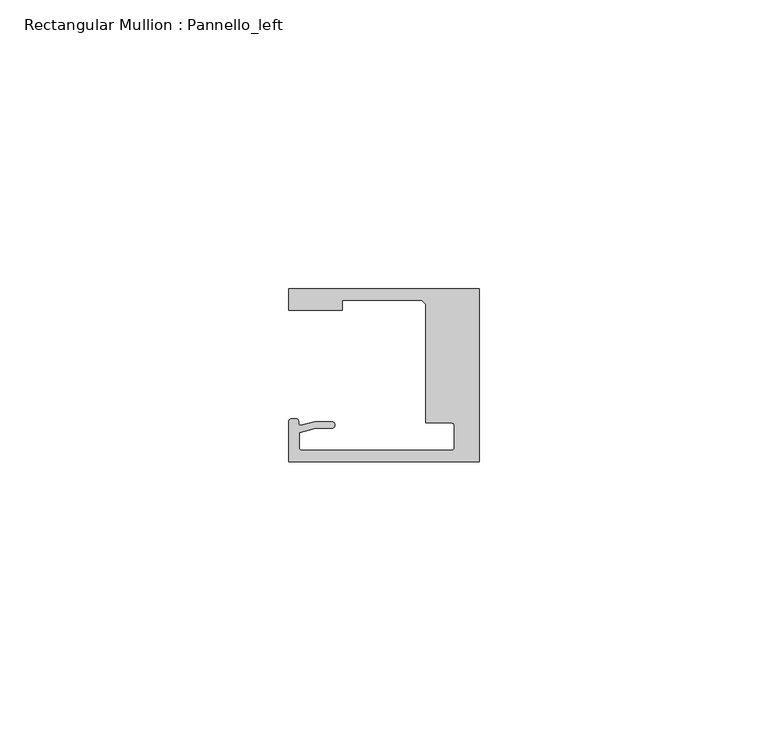
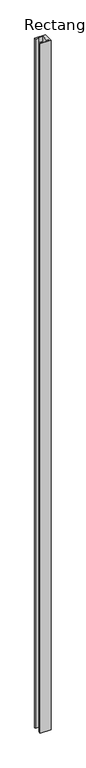
"""IFC4 building model written with IfcOpenShell, lengths in millimetres: member geometry, Rectangular Mullion : Pannello_left."""

import ifcopenshell
import ifcopenshell.guid

model = None  # the IFC model being written
_history = None  # IfcOwnerHistory: only IFC2X3 demands one
_inside = {}  # id of a spatial element -> (the spatial element, [elements in it])
_under = {}  # id of a project, library or spatial element -> (it, [spatial elements below it])
_declared = {}  # id of a project -> (the project, [libraries it declares])
_typed = {}  # id of a type object -> (the type object, [elements of that type])
_made_of = {}  # id of a material, layer set ... -> (it, [elements and type objects made of it])


def new_model(schema):
    """Start an empty IFC model of exactly this schema.

    Asked for "IFC4X3", IfcOpenShell would pick the latest addendum, in which some entities
    have other attributes; the version numbers below select the first issue.
    IFC2X3 requires an IfcOwnerHistory on every rooted entity: one is made here for all.
    """
    global model, _history
    if schema == "IFC4X3":
        model = ifcopenshell.file(schema_version=(4, 3, 0, 0))
    else:
        model = ifcopenshell.file(schema=schema)
    _inside.clear()
    _under.clear()
    _declared.clear()
    _typed.clear()
    _made_of.clear()
    _history = None
    if model.schema == "IFC2X3":
        org = make("IfcOrganization", Name="unknown")
        user = make(
            "IfcPersonAndOrganization",
            ThePerson=make("IfcPerson", FamilyName="unknown"),
            TheOrganization=org,
        )
        app = make(
            "IfcApplication",
            ApplicationDeveloper=org,
            Version="unknown",
            ApplicationFullName="unknown",
            ApplicationIdentifier="unknown",
        )
        _history = make(
            "IfcOwnerHistory",
            OwningUser=user,
            OwningApplication=app,
            ChangeAction="ADDED",
            CreationDate=0,
        )
    return model


def make(cls, **values):
    """One entity of the class cls with the attributes given. An attribute that is None is left unset."""
    return model.create_entity(
        cls, **{name: value for name, value in values.items() if value is not None}
    )


def rooted(cls, **values):
    """An entity with a GlobalId (a new one), such as an element, a storey or a relation."""
    return make(cls, GlobalId=ifcopenshell.guid.new(), OwnerHistory=_history, **values)


def si_unit(unit_type, name, prefix=None):
    """IfcSIUnit, for example si_unit("LENGTHUNIT", "METRE", prefix="MILLI")."""
    return make("IfcSIUnit", UnitType=unit_type, Prefix=prefix, Name=name)


def assignment(units):
    """IfcUnitAssignment: the units of a project."""
    return None if units is None else make("IfcUnitAssignment", Units=units)


def point(xyz):
    """IfcCartesianPoint."""
    return None if xyz is None else make("IfcCartesianPoint", Coordinates=xyz)


def direction(xyz):
    """IfcDirection."""
    return None if xyz is None else make("IfcDirection", DirectionRatios=xyz)


def frame(location, z_axis=None, x_axis=None):
    """IfcAxis2Placement3D, a coordinate frame: its origin and axes. An axis left out is left unset."""
    return make(
        "IfcAxis2Placement3D",
        Location=point(location),
        Axis=direction(z_axis),
        RefDirection=direction(x_axis),
    )


def origin():
    """The frame at (0, 0, 0) with its axes left unset."""
    return frame((0.0, 0.0, 0.0))


def place(relative_to, where):
    """IfcLocalPlacement: puts the frame where relative to a parent placement (None: the world)."""
    return make(
        "IfcLocalPlacement", PlacementRelTo=relative_to, RelativePlacement=where
    )


def context(
    kind, dimensions, precision=None, world=None, true_north=None, identifier=None
):
    """IfcGeometricRepresentationContext, for example the 3D "Model" context."""
    return make(
        "IfcGeometricRepresentationContext",
        ContextIdentifier=identifier,
        ContextType=kind,
        CoordinateSpaceDimension=dimensions,
        Precision=precision,
        WorldCoordinateSystem=world,
        TrueNorth=true_north,
    )


def project(units=None, contexts=None):
    """IfcProject with its units and contexts."""
    return rooted(
        "IfcProject",
        Name="project",
        RepresentationContexts=contexts,
        UnitsInContext=assignment(units),
    )


def spatial(cls, under=None, at=None, **own):
    """A site, building, storey or space (cls), placed at a placement, below another one or the project."""
    s = rooted(cls, ObjectPlacement=at, **own)
    if under is not None:
        _under.setdefault(under.id(), (under, []))[1].append(s)
    return s


def polyline(points):
    """IfcPolyline through the points."""
    return make("IfcPolyline", Points=[point(p) for p in points])


def circle_curve(where, radius):
    """IfcCircle in the frame where."""
    return make("IfcCircle", Position=where, Radius=radius)


def shape(context_of_items, identifier, shape_type, items):
    """IfcShapeRepresentation: the items that make up one representation, for example the "Body"."""
    return make(
        "IfcShapeRepresentation",
        ContextOfItems=context_of_items,
        RepresentationIdentifier=identifier,
        RepresentationType=shape_type,
        Items=items,
    )


def source(mapping_origin, context_of_items, identifier, shape_type, items):
    """IfcRepresentationMap: a shape defined once, which mapped items show again and again."""
    return make(
        "IfcRepresentationMap",
        MappingOrigin=mapping_origin,
        MappedRepresentation=shape(context_of_items, identifier, shape_type, items),
    )


def transform(
    local_origin,
    x_axis=None,
    y_axis=None,
    z_axis=None,
    scale=None,
    scale2=None,
    scale3=None,
    uniform=True,
):
    """IfcCartesianTransformationOperator3D, or its non-uniform kind. x_axis, y_axis, z_axis: its Axis1, 2, 3."""
    if uniform:
        return make(
            "IfcCartesianTransformationOperator3D",
            Axis1=direction(x_axis),
            Axis2=direction(y_axis),
            LocalOrigin=point(local_origin),
            Scale=scale,
            Axis3=direction(z_axis),
        )
    return make(
        "IfcCartesianTransformationOperator3DnonUniform",
        Axis1=direction(x_axis),
        Axis2=direction(y_axis),
        LocalOrigin=point(local_origin),
        Scale=scale,
        Axis3=direction(z_axis),
        Scale2=scale2,
        Scale3=scale3,
    )


def mapped(mapping_source, mapping_target):
    """IfcMappedItem: shows the shape of a source again, moved by a transform."""
    return make(
        "IfcMappedItem", MappingSource=mapping_source, MappingTarget=mapping_target
    )


def made_of(thing, what):
    """Note that an element or type object is made of a material, layer set ...; save() writes the relation."""
    if what is not None:
        _made_of.setdefault(what.id(), (what, []))[1].append(thing)
    return thing


def element(
    cls,
    number,
    at=None,
    inside=None,
    cuts=None,
    type_object=None,
    material=None,
    context=None,
    identifier="Body",
    shape_type=None,
    held_by="IfcProductDefinitionShape",
    body=None,
    shapes=None,
    **own,
):
    """One element of the class cls, such as IfcWall. Its Tag is "e" and its number.

    at: its placement. inside: the storey or other place that contains it. cuts: it is an
    opening in that element (IfcRelVoidsElement). A single representation is given by context,
    identifier, shape_type and body (its items); several are given by shapes. held_by: the class
    of the entity that holds the representations. save() writes the other relations.
    """
    e = rooted(cls, Tag="e%d" % number, ObjectPlacement=at, **own)
    if body is not None:
        shapes = [shape(context, identifier, shape_type, body)]
    if shapes is not None:
        e.Representation = make(held_by, Representations=shapes)
    if inside is not None:
        _inside.setdefault(inside.id(), (inside, []))[1].append(e)
    if cuts is not None:
        rooted(
            "IfcRelVoidsElement", RelatingBuildingElement=cuts, RelatedOpeningElement=e
        )
    if type_object is not None:
        _typed.setdefault(type_object.id(), (type_object, []))[1].append(e)
    return made_of(e, material)


def aggregate(whole, parts):
    """IfcRelAggregates: a whole, such as a stair, and the parts it consists of."""
    return rooted("IfcRelAggregates", RelatingObject=whole, RelatedObjects=parts)


def save(model, path):
    """Write the relations noted so far, then the file.

    IfcRelAggregates (storeys below a building ...), IfcRelContainedInSpatialStructure (elements
    in a storey), IfcRelDefinesByType, IfcRelAssociatesMaterial and IfcRelDeclares: one each for
    every whole, place, type object, material and project.
    """
    for whole, parts in _under.values():
        aggregate(whole, parts)
    for where, things in _inside.values():
        rooted(
            "IfcRelContainedInSpatialStructure",
            RelatedElements=things,
            RelatingStructure=where,
        )
    for kind, things in _typed.values():
        rooted("IfcRelDefinesByType", RelatedObjects=things, RelatingType=kind)
    for what, things in _made_of.values():
        rooted("IfcRelAssociatesMaterial", RelatedObjects=things, RelatingMaterial=what)
    for by, libraries in _declared.values():
        rooted("IfcRelDeclares", RelatingContext=by, RelatedDefinitions=libraries)
    model.write(path)


def plane_surface(at):
    """IfcPlane: the flat surface through the origin of the frame at, square to its z axis."""
    return make("IfcPlane", Position=at)


def cylinder_surface(at, radius):
    """IfcCylindricalSurface: all points at the distance radius from the z axis of the frame at."""
    return make("IfcCylindricalSurface", Position=at, Radius=radius)


def revolved_surface(curve, axis_point, axis_direction):
    """IfcSurfaceOfRevolution: the curve turned about the line through axis_point along axis_direction."""
    return make(
        "IfcSurfaceOfRevolution",
        SweptCurve=make("IfcArbitraryOpenProfileDef", ProfileType="CURVE", Curve=curve),
        AxisPosition=make("IfcAxis1Placement", Location=point(axis_point), Axis=direction(axis_direction)),
    )


def extruded_surface(curve, direction_of_extrusion, depth):
    """IfcSurfaceOfLinearExtrusion: the curve pushed along a direction by depth."""
    return make(
        "IfcSurfaceOfLinearExtrusion",
        SweptCurve=make("IfcArbitraryOpenProfileDef", ProfileType="CURVE", Curve=curve),
        ExtrudedDirection=direction(direction_of_extrusion),
        Depth=depth,
    )


def spline_curve(degree, points, multiplicities, knots, weights=None):
    """IfcBSplineCurveWithKnots; with weights, IfcRationalBSplineCurveWithKnots."""
    own = dict(
        Degree=degree,
        ControlPointsList=[point(p) for p in points],
        CurveForm="UNSPECIFIED",
        ClosedCurve=False,
        SelfIntersect=False,
        KnotMultiplicities=multiplicities,
        Knots=knots,
        KnotSpec="UNSPECIFIED",
    )
    if weights is None:
        return make("IfcBSplineCurveWithKnots", **own)
    return make("IfcRationalBSplineCurveWithKnots", WeightsData=weights, **own)


def advanced_brep(points, edges, surfaces, faces):
    """IfcAdvancedBrep: a solid bounded by faces that lie on surfaces and meet in shared edges.

    An edge is (start, end): straight between two places in points (the first is 0);
    or (start, end, curve); or (start, end, curve, False) where it runs against its curve.
    A face is (place in surfaces, loops), or (place, loops, False) where it looks against
    its surface's normal. A loop lists edges by number (the first is 1), with a minus sign
    where the edge is run from its end to its start. The first loop is the outer one.
    """
    corners = [point(p) for p in points]
    vertices = [make("IfcVertexPoint", VertexGeometry=c) for c in corners]
    made = []
    for start, end, *more in edges:
        made.append(
            make(
                "IfcEdgeCurve",
                EdgeStart=vertices[start],
                EdgeEnd=vertices[end],
                EdgeGeometry=more[0] if more else make("IfcPolyline", Points=[corners[start], corners[end]]),
                SameSense=more[1] if len(more) > 1 else True,
            )
        )
    hull = []
    for where, loops, *sense in faces:
        bounds = []
        for j, loop in enumerate(loops):
            ring = [make("IfcOrientedEdge", EdgeElement=made[abs(k) - 1], Orientation=k > 0) for k in loop]
            bounds.append(
                make(
                    "IfcFaceOuterBound" if j == 0 else "IfcFaceBound",
                    Bound=make("IfcEdgeLoop", EdgeList=ring),
                    Orientation=True,
                )
            )
        hull.append(make("IfcAdvancedFace", Bounds=bounds, FaceSurface=surfaces[where], SameSense=sense[0] if sense else True))
    return make("IfcAdvancedBrep", Outer=make("IfcClosedShell", CfsFaces=hull))


def rectangular_mullion_pannello_left_7b51982d(model_context):
    return source(origin(), model_context, "Body", "AdvancedBrep", [
        advanced_brep(
        [(-33.0, 15.0, 0.0), (-33.0, 11.3000004, 0.0), (-23.700041, 11.3000004, 0.0), (-23.700041, 13.0000004, 0.0), (-10.0000103, 13.0000004, 0.0), (-9.2999726, 12.2999849, 0.0), (-9.2999726, -8.2500595, 0.0), (-4.7999726, -8.2500595, 0.0), (-4.2999726, -8.7500595, 0.0), (-4.2999726, -12.50001, 0.0), (-4.7999726, -13.00001, 0.0), (-30.69998, -13.00001, 0.0), (-31.19998, -12.50001, 0.0), (-31.19998, -9.9657591, 0.0), (-28.3419477, -9.1999523, 0.0), (-25.59998, -9.1999523, 0.0), (-25.59998, -7.9999523, 0.0), (-28.4999305, -7.9999523, 0.0), (-30.9223017, -8.6490241, 0.0), (-33.0000135, -8.0000472, 0.0), (-33.0000135, -15.0, 0.0), (0.0, -15.0, 0.0), (0.0, 15.0, 0.0), (-33.0, 15.0, -2260.0), (0.0, 15.0, -2260.0), (0.0, -15.0, -2260.0), (-33.0000135, -15.0, -2260.0), (-33.0000135, -8.0000472, -2260.0), (-30.9223017, -8.6490241, -2260.0), (-28.4999305, -7.9999523, -2260.0), (-25.59998, -7.9999523, -2260.0), (-25.59998, -9.1999523, -2260.0), (-28.3419477, -9.1999523, -2260.0), (-31.19998, -9.9657591, -2260.0), (-31.19998, -12.50001, -2260.0), (-30.69998, -13.00001, -2260.0), (-4.7999726, -13.00001, -2260.0), (-4.2999726, -12.50001, -2260.0), (-4.2999726, -8.7500595, -2260.0), (-4.7999726, -8.2500595, -2260.0), (-9.2999726, -8.2500595, -2260.0), (-9.2999726, 12.2999849, -2260.0), (-10.0000103, 13.0000004, -2260.0), (-23.700041, 13.0000004, -2260.0), (-23.700041, 11.3000004, -2260.0), (-33.0, 11.3000004, -2260.0)],
        [
            (0, 1),
            (1, 2),
            (2, 3),
            (3, 4),
            (4, 5),
            (5, 6),
            (6, 7),
            (7, 8, circle_curve(frame((-4.7999726, -8.7500595, 0.0), z_axis=(0.0, 0.0, -1.0), x_axis=(0.0, 1.0, 0.0)), 0.5)),
            (8, 9),
            (9, 10, circle_curve(frame((-4.7999726, -12.50001, 0.0), z_axis=(0.0, 0.0, -1.0), x_axis=(1.0, 0.0, 0.0)), 0.5)),
            (10, 11),
            (11, 12, circle_curve(frame((-30.69998, -12.50001, 0.0), z_axis=(0.0, 0.0, -1.0), x_axis=(0.0, -1.0, 0.0)), 0.5)),
            (12, 13),
            (13, 14),
            (14, 15),
            (15, 16, circle_curve(frame((-25.59998, -8.5999523, 0.0), z_axis=(0.0, 0.0, 1.0), x_axis=(0.0, -1.0, 0.0)), 0.6)),
            (16, 17),
            (17, 18),
            (18, 19, spline_curve(3, [(-30.9223017, -8.6490241, 0.0), (-31.312054066, -8.717747958, 0.0), (-31.298563602, -8.366228555, 0.0), (-31.305645054, -7.690065204, 0.0), (-31.357433266, -7.563996614, 0.0), (-32.262327879, -7.456527435, 0.0), (-33.0000135, -7.457047519, 0.0), (-33.0000135, -8.0000472, 0.0)], [4, 2, 2, 4], [0.0, 0.001840817752199412, 0.004996616814974408, 0.007702013405570312])),
            (19, 20),
            (20, 21),
            (21, 22),
            (22, 0),
            (23, 24),
            (24, 25),
            (25, 26),
            (26, 27),
            (27, 28, spline_curve(3, [(-33.0000135, -8.0000472, -2260.0), (-33.0000135, -7.457047519, -2260.0), (-32.262327879, -7.456527435, -2260.0), (-31.357433266, -7.563996614, -2260.0), (-31.305645054, -7.690065204, -2260.0), (-31.298563602, -8.366228555, -2260.0), (-31.312054066, -8.717747958, -2260.0), (-30.9223017, -8.6490241, -2260.0)], [4, 2, 2, 4], [0.0, 0.0027053965905959043, 0.0058611956533709, 0.007702013405570312])),
            (28, 29),
            (29, 30),
            (30, 31, circle_curve(frame((-25.59998, -8.5999523, -2260.0), z_axis=(0.0, 0.0, -1.0), x_axis=(0.0, -1.0, 0.0)), 0.6)),
            (31, 32),
            (32, 33),
            (33, 34),
            (34, 35, circle_curve(frame((-30.69998, -12.50001, -2260.0), z_axis=(0.0, 0.0, 1.0), x_axis=(0.0, -1.0, 0.0)), 0.5)),
            (35, 36),
            (36, 37, circle_curve(frame((-4.7999726, -12.50001, -2260.0), z_axis=(0.0, 0.0, 1.0), x_axis=(1.0, 0.0, 0.0)), 0.5)),
            (37, 38),
            (38, 39, circle_curve(frame((-4.7999726, -8.7500595, -2260.0), z_axis=(0.0, 0.0, 1.0), x_axis=(0.0, 1.0, 0.0)), 0.5)),
            (39, 40),
            (40, 41),
            (41, 42),
            (42, 43),
            (43, 44),
            (44, 45),
            (45, 23),
            (0, 23),
            (45, 1),
            (44, 2),
            (43, 3),
            (42, 4),
            (41, 5),
            (40, 6),
            (39, 7),
            (38, 8),
            (37, 9),
            (36, 10),
            (35, 11),
            (34, 12),
            (33, 13),
            (32, 14),
            (31, 15),
            (30, 16),
            (29, 17),
            (28, 18),
            (27, 19),
            (26, 20),
            (25, 21),
            (24, 22),
        ],
        [
            plane_surface(frame((0.0, -36.2491502, 0.0), z_axis=(0.0, 0.0, 1.0), x_axis=(-1.0, 0.0, 0.0))),
            plane_surface(frame((0.0, -36.2491502, -2260.0), z_axis=(0.0, 0.0, -1.0), x_axis=(-1.0, 0.0, 0.0))),
            plane_surface(frame((-33.0, 15.0, 0.0), z_axis=(-1.0, 0.0, 0.0), x_axis=(0.0, 0.0, -1.0))),
            plane_surface(frame((-33.0, 11.3000004, 0.0), z_axis=(0.0, -1.0, 0.0), x_axis=(0.0, 0.0, -1.0))),
            plane_surface(frame((-23.700041, 11.3000004, 0.0), z_axis=(1.0, 0.0, 0.0), x_axis=(0.0, 0.0, -1.0))),
            plane_surface(frame((-23.700041, 13.0000004, 0.0), z_axis=(0.0, -1.0, 0.0), x_axis=(0.0, 0.0, -1.0))),
            plane_surface(frame((-10.0000103, 13.0000004, 0.0), z_axis=(-0.7070955486277984, -0.7071180135668678, 0.0), x_axis=(0.0, 0.0, -1.0))),
            plane_surface(frame((-9.2999726, 12.2999849, 0.0), z_axis=(-1.0, 0.0, 0.0), x_axis=(0.0, 0.0, -1.0))),
            plane_surface(frame((-9.2999726, -8.2500595, 0.0), z_axis=(0.0, -1.0, 0.0), x_axis=(0.0, 0.0, -1.0))),
            revolved_surface(polyline([(-4.7999726, -8.2500595, -2260.0), (-4.7999726, -8.2500595, 0.0)]), (-4.7999726, -8.7500595, 0.0), (0.0, 0.0, -1.0)),
            plane_surface(frame((-4.2999726, -8.7500595, 0.0), z_axis=(-1.0, 0.0, 0.0), x_axis=(0.0, 0.0, -1.0))),
            revolved_surface(polyline([(-4.2999726, -12.50001, -2260.0), (-4.2999726, -12.50001, 0.0)]), (-4.7999726, -12.50001, 0.0), (0.0, 0.0, -1.0)),
            plane_surface(frame((-4.7999726, -13.00001, 0.0), z_axis=(0.0, 1.0, 0.0), x_axis=(0.0, 0.0, -1.0))),
            revolved_surface(polyline([(-30.69998, -13.00001, -2260.0), (-30.69998, -13.00001, 0.0)]), (-30.69998, -12.50001, 0.0), (0.0, 0.0, -1.0)),
            plane_surface(frame((-31.19998, -12.50001, 0.0), z_axis=(1.0, 0.0, 0.0), x_axis=(0.0, 0.0, -1.0))),
            plane_surface(frame((-31.19998, -9.9657591, 0.0), z_axis=(0.25881883204288636, -0.9659258833782002, 0.0), x_axis=(0.0, 0.0, -1.0))),
            plane_surface(frame((-28.3419477, -9.1999523, 0.0), z_axis=(0.0, -1.0, 0.0), x_axis=(0.0, 0.0, -1.0))),
            cylinder_surface(frame((-25.59998, -8.5999523, 0.0), z_axis=(0.0, 0.0, 1.0), x_axis=(0.0, -1.0, 0.0)), 0.6),
            plane_surface(frame((-25.59998, -7.9999523, 0.0), z_axis=(0.0, 1.0, 0.0), x_axis=(0.0, 0.0, -1.0))),
            plane_surface(frame((-28.4999305, -7.9999523, 0.0), z_axis=(-0.25881883200192934, 0.9659258833891746, 0.0), x_axis=(0.0, 0.0, -1.0))),
            extruded_surface(spline_curve(3, [(-30.9223017, -8.6490241, -2260.0), (-31.312054066, -8.717747958, -2260.0), (-31.298563602, -8.366228555, -2260.0), (-31.305645054, -7.690065204, -2260.0), (-31.357433266, -7.563996614, -2260.0), (-32.262327879, -7.456527435, -2260.0), (-33.0000135, -7.457047519, -2260.0), (-33.0000135, -8.0000472, -2260.0)], [4, 2, 2, 4], [0.0, 0.001840817752199412, 0.004996616814974408, 0.007702013405570312]), (0.0, 0.0, 2260.0), 2260.0),
            plane_surface(frame((-33.0000135, -8.0000472, 0.0), z_axis=(-1.0, 0.0, 0.0), x_axis=(0.0, 0.0, -1.0))),
            plane_surface(frame((-33.0000135, -15.0, 0.0), z_axis=(0.0, -1.0, 0.0), x_axis=(0.0, 0.0, -1.0))),
            plane_surface(frame((0.0, -15.0, 0.0), z_axis=(1.0, 0.0, 0.0), x_axis=(0.0, 0.0, -1.0))),
            plane_surface(frame((0.0, 15.0, 0.0), z_axis=(0.0, 1.0, 0.0), x_axis=(0.0, 0.0, -1.0))),
        ],
        [
            (0, [[1, 2, 3, 4, 5, 6, 7, 8, 9, 10, 11, 12, 13, 14, 15, 16, 17, 18, 19, 20, 21, 22, 23]]),
            (1, [[24, 25, 26, 27, 28, 29, 30, 31, 32, 33, 34, 35, 36, 37, 38, 39, 40, 41, 42, 43, 44, 45, 46]]),
            (2, [[-1, 47, -46, 48]]),
            (3, [[-2, -48, -45, 49]]),
            (4, [[-3, -49, -44, 50]]),
            (5, [[-4, -50, -43, 51]]),
            (6, [[-5, -51, -42, 52]]),
            (7, [[-6, -52, -41, 53]]),
            (8, [[-7, -53, -40, 54]]),
            (9, [[-8, -54, -39, 55]]),
            (10, [[-9, -55, -38, 56]]),
            (11, [[-10, -56, -37, 57]]),
            (12, [[-11, -57, -36, 58]]),
            (13, [[-12, -58, -35, 59]]),
            (14, [[-13, -59, -34, 60]]),
            (15, [[-14, -60, -33, 61]]),
            (16, [[-15, -61, -32, 62]]),
            (17, [[-16, -62, -31, 63]]),
            (18, [[-17, -63, -30, 64]]),
            (19, [[-18, -64, -29, 65]]),
            (20, [[-19, -65, -28, 66]]),
            (21, [[-20, -66, -27, 67]]),
            (22, [[-21, -67, -26, 68]]),
            (23, [[-22, -68, -25, 69]]),
            (24, [[-23, -69, -24, -47]]),
        ],
    ),
    ])


if __name__ == "__main__":
    model = new_model("IFC4")
    model_context = context("Model", 3, world=origin())
    ifc_project = project(units=[si_unit("LENGTHUNIT", "METRE", prefix="MILLI")], contexts=[model_context])
    site = spatial("IfcSite", under=ifc_project)
    building = spatial("IfcBuilding", under=site)
    placement = place(None, origin())
    rectangular_mullion_pannello_left_shape = rectangular_mullion_pannello_left_7b51982d(model_context)
    element("IfcMember", 1, ObjectType="Rectangular Mullion : Pannello_left", at=placement, inside=building, context=model_context, shape_type="MappedRepresentation", body=[
        mapped(rectangular_mullion_pannello_left_shape, transform((0.0, 0.0, 0.0), x_axis=(1.0, 0.0, 0.0), y_axis=(0.0, 1.0, 0.0), z_axis=(0.0, 0.0, 1.0))),
    ])
    save(model, "model.ifc")

# Revit data of these elements
# Type "Rectangular Mullion : Pannello_left"
#   built-in parameter 1007322 = 0.0984252 (stored number, unit not read)
#   built-in parameter 1007320 = 0.0305117 (stored number, unit not read)
